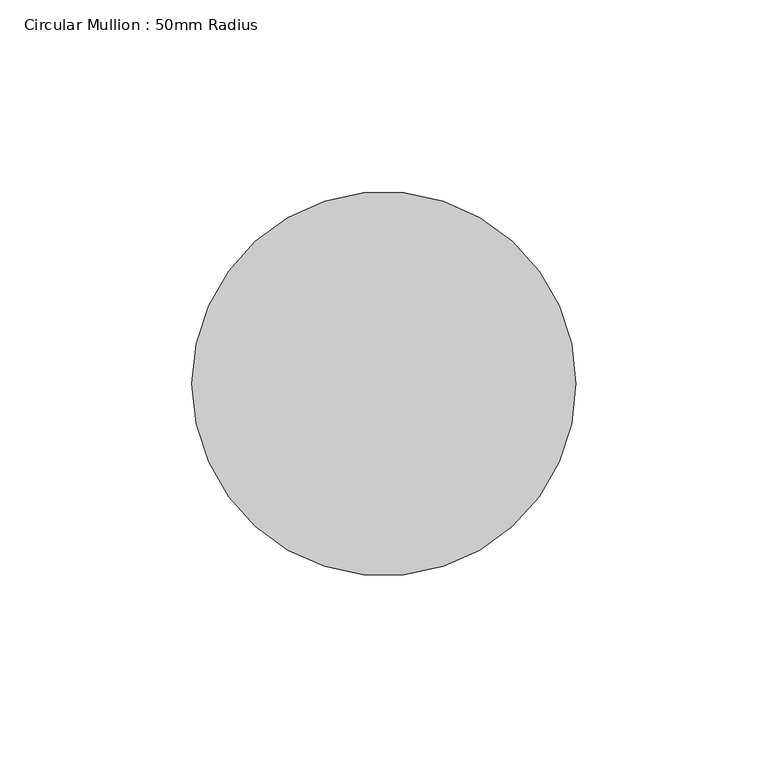
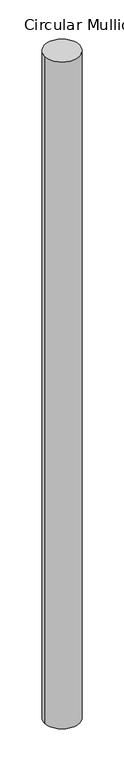
"""IFC4 building model written with IfcOpenShell, lengths in millimetres: member geometry, Circular Mullion : 50mm Radius."""

from ifc_helpers import new_model, si_unit, point, frame, frame_2d, origin, place, context, project, spatial, circle_curve, trimmed, segment, composite_curve, outline, extrude, source, transform, mapped, element, save


def circular_mullion_50mm_radius_b2d07eb4(model_context):
    return source(origin(), model_context, "Body", "SweptSolid", [
        extrude(outline(composite_curve([segment(trimmed(circle_curve(frame_2d((-50.0, 0.0)), 50.0), [point((0.0, 0.0))], [point((-100.0, 0.0))], False, "CARTESIAN"), True, "CONTINUOUS"), segment(trimmed(circle_curve(frame_2d((-50.0, 0.0)), 50.0), [point((-100.0, 0.0))], [point((0.0, 0.0))], False, "CARTESIAN"), True, "CONTINUOUS")], self_intersect=False)), frame((0.0, 0.0, -2034.2259818), z_axis=(0.0, 0.0, 1.0), x_axis=(1.0, 0.0, 0.0)), (0.0, 0.0, 1.0), 2034.2259818),
    ])


if __name__ == "__main__":
    model = new_model("IFC4")
    model_context = context("Model", 3, world=origin())
    ifc_project = project(units=[si_unit("LENGTHUNIT", "METRE", prefix="MILLI")], contexts=[model_context])
    site = spatial("IfcSite", under=ifc_project)
    building = spatial("IfcBuilding", under=site)
    placement = place(None, origin())
    circular_mullion_50mm_radius_shape = circular_mullion_50mm_radius_b2d07eb4(model_context)
    element("IfcMember", 1, ObjectType="Circular Mullion : 50mm Radius", at=placement, inside=building, context=model_context, shape_type="MappedRepresentation", body=[
        mapped(circular_mullion_50mm_radius_shape, transform((0.0, 0.0, 0.0), x_axis=(1.0, 0.0, 0.0), y_axis=(0.0, 1.0, 0.0), z_axis=(0.0, 0.0, 1.0))),
    ])
    save(model, "model.ifc")

# Revit data of these elements
# Type "Circular Mullion : 50mm Radius"
#   built-in parameter 1007350 = 0.164042 (stored number, unit not read)
# Element 1 (IfcMember, "Circular Mullion : 50mm Radius")
#   Materials on its faces: "Aluminium"
# Materials
#   "Aluminium": class "Metal", colour RGB 247 247 247, transparency 0, Description = "Aluminium 6061", Cost = 0
